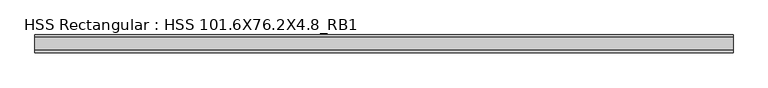
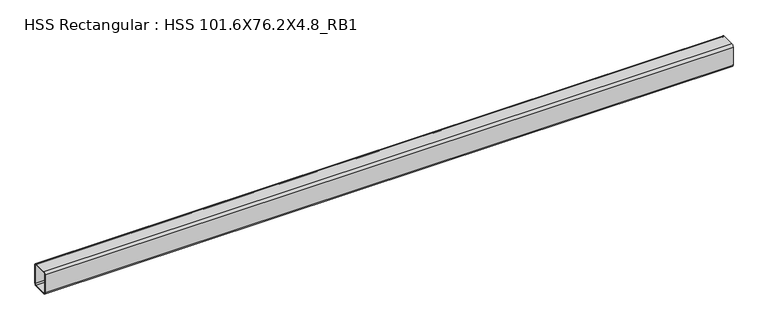
"""IFC4 building model written with IfcOpenShell, lengths in millimetres: beam geometry, HSS Rectangular : HSS 101.6X76.2X4.8_RB1."""

import ifcopenshell
import ifcopenshell.guid

model = None  # the IFC model being written
_history = None  # IfcOwnerHistory: only IFC2X3 demands one
_inside = {}  # id of a spatial element -> (the spatial element, [elements in it])
_under = {}  # id of a project, library or spatial element -> (it, [spatial elements below it])
_declared = {}  # id of a project -> (the project, [libraries it declares])
_typed = {}  # id of a type object -> (the type object, [elements of that type])
_made_of = {}  # id of a material, layer set ... -> (it, [elements and type objects made of it])


def new_model(schema):
    """Start an empty IFC model of exactly this schema.

    Asked for "IFC4X3", IfcOpenShell would pick the latest addendum, in which some entities
    have other attributes; the version numbers below select the first issue.
    IFC2X3 requires an IfcOwnerHistory on every rooted entity: one is made here for all.
    """
    global model, _history
    if schema == "IFC4X3":
        model = ifcopenshell.file(schema_version=(4, 3, 0, 0))
    else:
        model = ifcopenshell.file(schema=schema)
    _inside.clear()
    _under.clear()
    _declared.clear()
    _typed.clear()
    _made_of.clear()
    _history = None
    if model.schema == "IFC2X3":
        org = make("IfcOrganization", Name="unknown")
        user = make(
            "IfcPersonAndOrganization",
            ThePerson=make("IfcPerson", FamilyName="unknown"),
            TheOrganization=org,
        )
        app = make(
            "IfcApplication",
            ApplicationDeveloper=org,
            Version="unknown",
            ApplicationFullName="unknown",
            ApplicationIdentifier="unknown",
        )
        _history = make(
            "IfcOwnerHistory",
            OwningUser=user,
            OwningApplication=app,
            ChangeAction="ADDED",
            CreationDate=0,
        )
    return model


def make(cls, **values):
    """One entity of the class cls with the attributes given. An attribute that is None is left unset."""
    return model.create_entity(
        cls, **{name: value for name, value in values.items() if value is not None}
    )


def rooted(cls, **values):
    """An entity with a GlobalId (a new one), such as an element, a storey or a relation."""
    return make(cls, GlobalId=ifcopenshell.guid.new(), OwnerHistory=_history, **values)


def si_unit(unit_type, name, prefix=None):
    """IfcSIUnit, for example si_unit("LENGTHUNIT", "METRE", prefix="MILLI")."""
    return make("IfcSIUnit", UnitType=unit_type, Prefix=prefix, Name=name)


def assignment(units):
    """IfcUnitAssignment: the units of a project."""
    return None if units is None else make("IfcUnitAssignment", Units=units)


def point(xyz):
    """IfcCartesianPoint."""
    return None if xyz is None else make("IfcCartesianPoint", Coordinates=xyz)


def direction(xyz):
    """IfcDirection."""
    return None if xyz is None else make("IfcDirection", DirectionRatios=xyz)


def frame(location, z_axis=None, x_axis=None):
    """IfcAxis2Placement3D, a coordinate frame: its origin and axes. An axis left out is left unset."""
    return make(
        "IfcAxis2Placement3D",
        Location=point(location),
        Axis=direction(z_axis),
        RefDirection=direction(x_axis),
    )


def frame_2d(location, x_axis=None):
    """IfcAxis2Placement2D, a coordinate frame in the plane: its origin and x axis."""
    return make(
        "IfcAxis2Placement2D", Location=point(location), RefDirection=direction(x_axis)
    )


def origin():
    """The frame at (0, 0, 0) with its axes left unset."""
    return frame((0.0, 0.0, 0.0))


def place(relative_to, where):
    """IfcLocalPlacement: puts the frame where relative to a parent placement (None: the world)."""
    return make(
        "IfcLocalPlacement", PlacementRelTo=relative_to, RelativePlacement=where
    )


def context(
    kind, dimensions, precision=None, world=None, true_north=None, identifier=None
):
    """IfcGeometricRepresentationContext, for example the 3D "Model" context."""
    return make(
        "IfcGeometricRepresentationContext",
        ContextIdentifier=identifier,
        ContextType=kind,
        CoordinateSpaceDimension=dimensions,
        Precision=precision,
        WorldCoordinateSystem=world,
        TrueNorth=true_north,
    )


def project(units=None, contexts=None):
    """IfcProject with its units and contexts."""
    return rooted(
        "IfcProject",
        Name="project",
        RepresentationContexts=contexts,
        UnitsInContext=assignment(units),
    )


def spatial(cls, under=None, at=None, **own):
    """A site, building, storey or space (cls), placed at a placement, below another one or the project."""
    s = rooted(cls, ObjectPlacement=at, **own)
    if under is not None:
        _under.setdefault(under.id(), (under, []))[1].append(s)
    return s


def polyline(points):
    """IfcPolyline through the points."""
    return make("IfcPolyline", Points=[point(p) for p in points])


def circle_curve(where, radius):
    """IfcCircle in the frame where."""
    return make("IfcCircle", Position=where, Radius=radius)


def trimmed(basis, trim1, trim2, sense, master):
    """IfcTrimmedCurve: the piece of a basis curve between two trims."""
    return make(
        "IfcTrimmedCurve",
        BasisCurve=basis,
        Trim1=trim1,
        Trim2=trim2,
        SenseAgreement=sense,
        MasterRepresentation=master,
    )


def segment(curve, same_sense, transition):
    """IfcCompositeCurveSegment."""
    return make(
        "IfcCompositeCurveSegment",
        Transition=transition,
        SameSense=same_sense,
        ParentCurve=curve,
    )


def composite_curve(segments, self_intersect=None):
    """IfcCompositeCurve: segments joined end to end."""
    return make("IfcCompositeCurve", Segments=segments, SelfIntersect=self_intersect)


def outline(outer, holes=None, kind="AREA"):
    """IfcArbitraryClosedProfileDef: a profile drawn as a closed curve; with holes, ...WithVoids."""
    if holes is None:
        return make("IfcArbitraryClosedProfileDef", ProfileType=kind, OuterCurve=outer)
    return make(
        "IfcArbitraryProfileDefWithVoids",
        ProfileType=kind,
        OuterCurve=outer,
        InnerCurves=holes,
    )


def extrude(swept, where, along, depth):
    """IfcExtrudedAreaSolid: the profile swept, set in the frame where, extruded along a direction by depth."""
    return make(
        "IfcExtrudedAreaSolid",
        SweptArea=swept,
        Position=where,
        ExtrudedDirection=direction(along),
        Depth=depth,
    )


def shape(context_of_items, identifier, shape_type, items):
    """IfcShapeRepresentation: the items that make up one representation, for example the "Body"."""
    return make(
        "IfcShapeRepresentation",
        ContextOfItems=context_of_items,
        RepresentationIdentifier=identifier,
        RepresentationType=shape_type,
        Items=items,
    )


def source(mapping_origin, context_of_items, identifier, shape_type, items):
    """IfcRepresentationMap: a shape defined once, which mapped items show again and again."""
    return make(
        "IfcRepresentationMap",
        MappingOrigin=mapping_origin,
        MappedRepresentation=shape(context_of_items, identifier, shape_type, items),
    )


def transform(
    local_origin,
    x_axis=None,
    y_axis=None,
    z_axis=None,
    scale=None,
    scale2=None,
    scale3=None,
    uniform=True,
):
    """IfcCartesianTransformationOperator3D, or its non-uniform kind. x_axis, y_axis, z_axis: its Axis1, 2, 3."""
    if uniform:
        return make(
            "IfcCartesianTransformationOperator3D",
            Axis1=direction(x_axis),
            Axis2=direction(y_axis),
            LocalOrigin=point(local_origin),
            Scale=scale,
            Axis3=direction(z_axis),
        )
    return make(
        "IfcCartesianTransformationOperator3DnonUniform",
        Axis1=direction(x_axis),
        Axis2=direction(y_axis),
        LocalOrigin=point(local_origin),
        Scale=scale,
        Axis3=direction(z_axis),
        Scale2=scale2,
        Scale3=scale3,
    )


def mapped(mapping_source, mapping_target):
    """IfcMappedItem: shows the shape of a source again, moved by a transform."""
    return make(
        "IfcMappedItem", MappingSource=mapping_source, MappingTarget=mapping_target
    )


def made_of(thing, what):
    """Note that an element or type object is made of a material, layer set ...; save() writes the relation."""
    if what is not None:
        _made_of.setdefault(what.id(), (what, []))[1].append(thing)
    return thing


def element(
    cls,
    number,
    at=None,
    inside=None,
    cuts=None,
    type_object=None,
    material=None,
    context=None,
    identifier="Body",
    shape_type=None,
    held_by="IfcProductDefinitionShape",
    body=None,
    shapes=None,
    **own,
):
    """One element of the class cls, such as IfcWall. Its Tag is "e" and its number.

    at: its placement. inside: the storey or other place that contains it. cuts: it is an
    opening in that element (IfcRelVoidsElement). A single representation is given by context,
    identifier, shape_type and body (its items); several are given by shapes. held_by: the class
    of the entity that holds the representations. save() writes the other relations.
    """
    e = rooted(cls, Tag="e%d" % number, ObjectPlacement=at, **own)
    if body is not None:
        shapes = [shape(context, identifier, shape_type, body)]
    if shapes is not None:
        e.Representation = make(held_by, Representations=shapes)
    if inside is not None:
        _inside.setdefault(inside.id(), (inside, []))[1].append(e)
    if cuts is not None:
        rooted(
            "IfcRelVoidsElement", RelatingBuildingElement=cuts, RelatedOpeningElement=e
        )
    if type_object is not None:
        _typed.setdefault(type_object.id(), (type_object, []))[1].append(e)
    return made_of(e, material)


def aggregate(whole, parts):
    """IfcRelAggregates: a whole, such as a stair, and the parts it consists of."""
    return rooted("IfcRelAggregates", RelatingObject=whole, RelatedObjects=parts)


def save(model, path):
    """Write the relations noted so far, then the file.

    IfcRelAggregates (storeys below a building ...), IfcRelContainedInSpatialStructure (elements
    in a storey), IfcRelDefinesByType, IfcRelAssociatesMaterial and IfcRelDeclares: one each for
    every whole, place, type object, material and project.
    """
    for whole, parts in _under.values():
        aggregate(whole, parts)
    for where, things in _inside.values():
        rooted(
            "IfcRelContainedInSpatialStructure",
            RelatedElements=things,
            RelatingStructure=where,
        )
    for kind, things in _typed.values():
        rooted("IfcRelDefinesByType", RelatedObjects=things, RelatingType=kind)
    for what, things in _made_of.values():
        rooted("IfcRelAssociatesMaterial", RelatedObjects=things, RelatingMaterial=what)
    for by, libraries in _declared.values():
        rooted("IfcRelDeclares", RelatingContext=by, RelatedDefinitions=libraries)
    model.write(path)


def hss_rectangular_hss_101_6x76_2x4_8_rb1_a6ff69d1(model_context):
    return source(origin(), model_context, "Body", "SweptSolid", [
        extrude(outline(composite_curve([segment(trimmed(circle_curve(frame_2d((-28.575, 41.275)), 9.525), [point((-38.1, 41.275))], [point((-28.575, 50.8))], False, "CARTESIAN"), True, "CONTINUOUS"), segment(polyline([(-28.575, 50.8), (28.575, 50.8)]), True, "CONTINUOUS"), segment(trimmed(circle_curve(frame_2d((28.575, 41.275)), 9.525), [point((28.575, 50.8))], [point((38.1, 41.275))], False, "CARTESIAN"), True, "CONTINUOUS"), segment(polyline([(38.1, 41.275), (38.1, -41.275)]), True, "CONTINUOUS"), segment(trimmed(circle_curve(frame_2d((28.575, -41.275)), 9.525), [point((38.1, -41.275))], [point((28.575, -50.8))], False, "CARTESIAN"), True, "CONTINUOUS"), segment(polyline([(28.575, -50.8), (-28.575, -50.8)]), True, "CONTINUOUS"), segment(trimmed(circle_curve(frame_2d((-28.575, -41.275)), 9.525), [point((-28.575, -50.8))], [point((-38.1, -41.275))], False, "CARTESIAN"), True, "CONTINUOUS"), segment(polyline([(-38.1, -41.275), (-38.1, 41.275)]), True, "CONTINUOUS")], self_intersect=False), holes=[composite_curve([segment(polyline([(28.575, 46.0375), (-28.575, 46.0375)]), True, "CONTINUOUS"), segment(trimmed(circle_curve(frame_2d((-28.575, 41.275)), 4.7625), [point((-28.575, 46.0375))], [point((-33.3375, 41.275))], True, "CARTESIAN"), True, "CONTINUOUS"), segment(polyline([(-33.3375, 41.275), (-33.3375, -41.275)]), True, "CONTINUOUS"), segment(trimmed(circle_curve(frame_2d((-28.575, -41.275)), 4.7625), [point((-33.3375, -41.275))], [point((-28.575, -46.0375))], True, "CARTESIAN"), True, "CONTINUOUS"), segment(polyline([(-28.575, -46.0375), (28.575, -46.0375)]), True, "CONTINUOUS"), segment(trimmed(circle_curve(frame_2d((28.575, -41.275)), 4.7625), [point((28.575, -46.0375))], [point((33.3375, -41.275))], True, "CARTESIAN"), True, "CONTINUOUS"), segment(polyline([(33.3375, -41.275), (33.3375, 41.275)]), True, "CONTINUOUS"), segment(trimmed(circle_curve(frame_2d((28.575, 41.275)), 4.7625), [point((33.3375, 41.275))], [point((28.575, 46.0375))], True, "CARTESIAN"), True, "CONTINUOUS")], self_intersect=False)]), frame((-1527.8674477, 0.0, 0.0), z_axis=(1.0, 0.0, 0.0), x_axis=(0.0, 1.0, 0.0)), (0.0, 0.0, 1.0), 2987.3000012),
    ])


if __name__ == "__main__":
    model = new_model("IFC4")
    model_context = context("Model", 3, world=origin())
    ifc_project = project(units=[si_unit("LENGTHUNIT", "METRE", prefix="MILLI")], contexts=[model_context])
    site = spatial("IfcSite", under=ifc_project)
    building = spatial("IfcBuilding", under=site)
    placement = place(None, origin())
    hss_rectangular_hss_101_6x76_2x4_8_rb1_shape = hss_rectangular_hss_101_6x76_2x4_8_rb1_a6ff69d1(model_context)
    element("IfcBeam", 1, ObjectType="HSS Rectangular : HSS 101.6X76.2X4.8_RB1", at=placement, inside=building, context=model_context, shape_type="MappedRepresentation", body=[
        mapped(hss_rectangular_hss_101_6x76_2x4_8_rb1_shape, transform((0.0, 0.0, 0.0), x_axis=(1.0, 0.0, 0.0), y_axis=(0.0, 1.0, 0.0), z_axis=(0.0, 0.0, 1.0))),
    ])
    save(model, "model.ifc")

# Revit data of these elements
# Type "HSS Rectangular : HSS 101.6X76.2X4.8_RB1"
#   Section Name Key = "HSS 4X3X3/16"
#   Assembly Code = "B10"
#   Width = 7.62 cm
#   Wall Nominal Thickness = 0.4763 cm
#   Wall Design Thickness = 0.442 cm
#   Torsional Moment of Inertia = 260.561 cm⁴
#   Torsional Modulus = 61.2876 cm³
#   Section Area = 14.4516 cm²
#   Plastic Modulus weak axis = 40.3122 cm³
#   Plastic Modulus strong axis = 49.1612 cm³
#   Perimeter = 0.881482 m²/m
#   Outer Fillet = 0.9525 cm
#   Nominal Weight = 12.1285 kgf/m
#   Moment of Inertia weak axis = 131.529 cm⁴
#   Moment of Inertia strong axis = 205.202 cm⁴
#   Inner Fillet = 0.4763 cm
#   Height = 10.16 cm
#   Elastic Modulus weak axis = 34.4128 cm³
#   Elastic Modulus strong axis = 40.476 cm³
#   Centroid Vertical = 5.08 cm
#   Centroid Horizontal = 3.81 cm
#   Length [instance default] = 1524 mm
#   Structural Material [instance default] = Steel ASTM A500, Grade B, Rectangular and Square
#   Principal Axes Angle = 0
# Element 1 (IfcBeam, "HSS Rectangular : HSS 101.6X76.2X4.8_RB1")
#   Structural Material = Steel ASTM A992
#   Materials on its faces: "Steel ASTM A992"
# Materials
#   "Steel ASTM A500, Grade B, Rectangular and Square": class "Metal", colour RGB 199 199 199, transparency 0, Description = "Carbon steel", Cost = 0
#   "Steel ASTM A992": class "Metal", colour RGB 199 199 199, transparency 0, Description = "Structural steel 50ksi", Cost = 0
